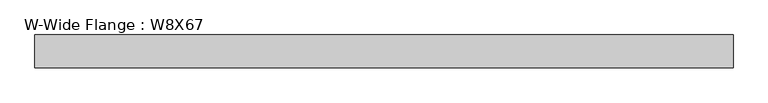
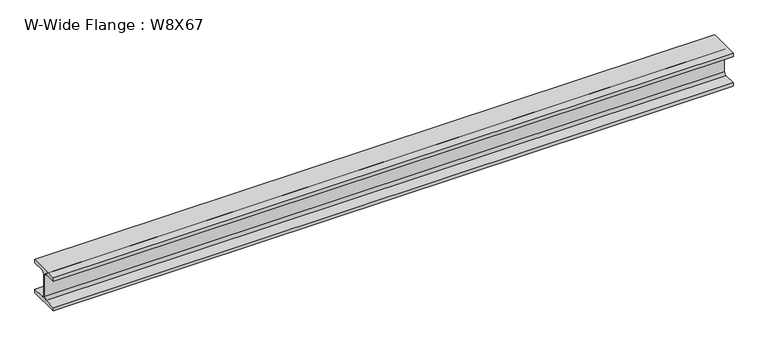
"""IFC4 building model written with IfcOpenShell, lengths in millimetres: beam geometry, W-Wide Flange : W8X67."""

import ifcopenshell
import ifcopenshell.guid

model = None  # the IFC model being written
_history = None  # IfcOwnerHistory: only IFC2X3 demands one
_inside = {}  # id of a spatial element -> (the spatial element, [elements in it])
_under = {}  # id of a project, library or spatial element -> (it, [spatial elements below it])
_declared = {}  # id of a project -> (the project, [libraries it declares])
_typed = {}  # id of a type object -> (the type object, [elements of that type])
_made_of = {}  # id of a material, layer set ... -> (it, [elements and type objects made of it])


def new_model(schema):
    """Start an empty IFC model of exactly this schema.

    Asked for "IFC4X3", IfcOpenShell would pick the latest addendum, in which some entities
    have other attributes; the version numbers below select the first issue.
    IFC2X3 requires an IfcOwnerHistory on every rooted entity: one is made here for all.
    """
    global model, _history
    if schema == "IFC4X3":
        model = ifcopenshell.file(schema_version=(4, 3, 0, 0))
    else:
        model = ifcopenshell.file(schema=schema)
    _inside.clear()
    _under.clear()
    _declared.clear()
    _typed.clear()
    _made_of.clear()
    _history = None
    if model.schema == "IFC2X3":
        org = make("IfcOrganization", Name="unknown")
        user = make(
            "IfcPersonAndOrganization",
            ThePerson=make("IfcPerson", FamilyName="unknown"),
            TheOrganization=org,
        )
        app = make(
            "IfcApplication",
            ApplicationDeveloper=org,
            Version="unknown",
            ApplicationFullName="unknown",
            ApplicationIdentifier="unknown",
        )
        _history = make(
            "IfcOwnerHistory",
            OwningUser=user,
            OwningApplication=app,
            ChangeAction="ADDED",
            CreationDate=0,
        )
    return model


def make(cls, **values):
    """One entity of the class cls with the attributes given. An attribute that is None is left unset."""
    return model.create_entity(
        cls, **{name: value for name, value in values.items() if value is not None}
    )


def rooted(cls, **values):
    """An entity with a GlobalId (a new one), such as an element, a storey or a relation."""
    return make(cls, GlobalId=ifcopenshell.guid.new(), OwnerHistory=_history, **values)


def si_unit(unit_type, name, prefix=None):
    """IfcSIUnit, for example si_unit("LENGTHUNIT", "METRE", prefix="MILLI")."""
    return make("IfcSIUnit", UnitType=unit_type, Prefix=prefix, Name=name)


def assignment(units):
    """IfcUnitAssignment: the units of a project."""
    return None if units is None else make("IfcUnitAssignment", Units=units)


def point(xyz):
    """IfcCartesianPoint."""
    return None if xyz is None else make("IfcCartesianPoint", Coordinates=xyz)


def direction(xyz):
    """IfcDirection."""
    return None if xyz is None else make("IfcDirection", DirectionRatios=xyz)


def frame(location, z_axis=None, x_axis=None):
    """IfcAxis2Placement3D, a coordinate frame: its origin and axes. An axis left out is left unset."""
    return make(
        "IfcAxis2Placement3D",
        Location=point(location),
        Axis=direction(z_axis),
        RefDirection=direction(x_axis),
    )


def frame_2d(location, x_axis=None):
    """IfcAxis2Placement2D, a coordinate frame in the plane: its origin and x axis."""
    return make(
        "IfcAxis2Placement2D", Location=point(location), RefDirection=direction(x_axis)
    )


def origin():
    """The frame at (0, 0, 0) with its axes left unset."""
    return frame((0.0, 0.0, 0.0))


def place(relative_to, where):
    """IfcLocalPlacement: puts the frame where relative to a parent placement (None: the world)."""
    return make(
        "IfcLocalPlacement", PlacementRelTo=relative_to, RelativePlacement=where
    )


def context(
    kind, dimensions, precision=None, world=None, true_north=None, identifier=None
):
    """IfcGeometricRepresentationContext, for example the 3D "Model" context."""
    return make(
        "IfcGeometricRepresentationContext",
        ContextIdentifier=identifier,
        ContextType=kind,
        CoordinateSpaceDimension=dimensions,
        Precision=precision,
        WorldCoordinateSystem=world,
        TrueNorth=true_north,
    )


def project(units=None, contexts=None):
    """IfcProject with its units and contexts."""
    return rooted(
        "IfcProject",
        Name="project",
        RepresentationContexts=contexts,
        UnitsInContext=assignment(units),
    )


def spatial(cls, under=None, at=None, **own):
    """A site, building, storey or space (cls), placed at a placement, below another one or the project."""
    s = rooted(cls, ObjectPlacement=at, **own)
    if under is not None:
        _under.setdefault(under.id(), (under, []))[1].append(s)
    return s


def polyline(points):
    """IfcPolyline through the points."""
    return make("IfcPolyline", Points=[point(p) for p in points])


def circle_curve(where, radius):
    """IfcCircle in the frame where."""
    return make("IfcCircle", Position=where, Radius=radius)


def trimmed(basis, trim1, trim2, sense, master):
    """IfcTrimmedCurve: the piece of a basis curve between two trims."""
    return make(
        "IfcTrimmedCurve",
        BasisCurve=basis,
        Trim1=trim1,
        Trim2=trim2,
        SenseAgreement=sense,
        MasterRepresentation=master,
    )


def segment(curve, same_sense, transition):
    """IfcCompositeCurveSegment."""
    return make(
        "IfcCompositeCurveSegment",
        Transition=transition,
        SameSense=same_sense,
        ParentCurve=curve,
    )


def composite_curve(segments, self_intersect=None):
    """IfcCompositeCurve: segments joined end to end."""
    return make("IfcCompositeCurve", Segments=segments, SelfIntersect=self_intersect)


def outline(outer, holes=None, kind="AREA"):
    """IfcArbitraryClosedProfileDef: a profile drawn as a closed curve; with holes, ...WithVoids."""
    if holes is None:
        return make("IfcArbitraryClosedProfileDef", ProfileType=kind, OuterCurve=outer)
    return make(
        "IfcArbitraryProfileDefWithVoids",
        ProfileType=kind,
        OuterCurve=outer,
        InnerCurves=holes,
    )


def extrude(swept, where, along, depth):
    """IfcExtrudedAreaSolid: the profile swept, set in the frame where, extruded along a direction by depth."""
    return make(
        "IfcExtrudedAreaSolid",
        SweptArea=swept,
        Position=where,
        ExtrudedDirection=direction(along),
        Depth=depth,
    )


def shape(context_of_items, identifier, shape_type, items):
    """IfcShapeRepresentation: the items that make up one representation, for example the "Body"."""
    return make(
        "IfcShapeRepresentation",
        ContextOfItems=context_of_items,
        RepresentationIdentifier=identifier,
        RepresentationType=shape_type,
        Items=items,
    )


def source(mapping_origin, context_of_items, identifier, shape_type, items):
    """IfcRepresentationMap: a shape defined once, which mapped items show again and again."""
    return make(
        "IfcRepresentationMap",
        MappingOrigin=mapping_origin,
        MappedRepresentation=shape(context_of_items, identifier, shape_type, items),
    )


def transform(
    local_origin,
    x_axis=None,
    y_axis=None,
    z_axis=None,
    scale=None,
    scale2=None,
    scale3=None,
    uniform=True,
):
    """IfcCartesianTransformationOperator3D, or its non-uniform kind. x_axis, y_axis, z_axis: its Axis1, 2, 3."""
    if uniform:
        return make(
            "IfcCartesianTransformationOperator3D",
            Axis1=direction(x_axis),
            Axis2=direction(y_axis),
            LocalOrigin=point(local_origin),
            Scale=scale,
            Axis3=direction(z_axis),
        )
    return make(
        "IfcCartesianTransformationOperator3DnonUniform",
        Axis1=direction(x_axis),
        Axis2=direction(y_axis),
        LocalOrigin=point(local_origin),
        Scale=scale,
        Axis3=direction(z_axis),
        Scale2=scale2,
        Scale3=scale3,
    )


def mapped(mapping_source, mapping_target):
    """IfcMappedItem: shows the shape of a source again, moved by a transform."""
    return make(
        "IfcMappedItem", MappingSource=mapping_source, MappingTarget=mapping_target
    )


def made_of(thing, what):
    """Note that an element or type object is made of a material, layer set ...; save() writes the relation."""
    if what is not None:
        _made_of.setdefault(what.id(), (what, []))[1].append(thing)
    return thing


def element(
    cls,
    number,
    at=None,
    inside=None,
    cuts=None,
    type_object=None,
    material=None,
    context=None,
    identifier="Body",
    shape_type=None,
    held_by="IfcProductDefinitionShape",
    body=None,
    shapes=None,
    **own,
):
    """One element of the class cls, such as IfcWall. Its Tag is "e" and its number.

    at: its placement. inside: the storey or other place that contains it. cuts: it is an
    opening in that element (IfcRelVoidsElement). A single representation is given by context,
    identifier, shape_type and body (its items); several are given by shapes. held_by: the class
    of the entity that holds the representations. save() writes the other relations.
    """
    e = rooted(cls, Tag="e%d" % number, ObjectPlacement=at, **own)
    if body is not None:
        shapes = [shape(context, identifier, shape_type, body)]
    if shapes is not None:
        e.Representation = make(held_by, Representations=shapes)
    if inside is not None:
        _inside.setdefault(inside.id(), (inside, []))[1].append(e)
    if cuts is not None:
        rooted(
            "IfcRelVoidsElement", RelatingBuildingElement=cuts, RelatedOpeningElement=e
        )
    if type_object is not None:
        _typed.setdefault(type_object.id(), (type_object, []))[1].append(e)
    return made_of(e, material)


def aggregate(whole, parts):
    """IfcRelAggregates: a whole, such as a stair, and the parts it consists of."""
    return rooted("IfcRelAggregates", RelatingObject=whole, RelatedObjects=parts)


def save(model, path):
    """Write the relations noted so far, then the file.

    IfcRelAggregates (storeys below a building ...), IfcRelContainedInSpatialStructure (elements
    in a storey), IfcRelDefinesByType, IfcRelAssociatesMaterial and IfcRelDeclares: one each for
    every whole, place, type object, material and project.
    """
    for whole, parts in _under.values():
        aggregate(whole, parts)
    for where, things in _inside.values():
        rooted(
            "IfcRelContainedInSpatialStructure",
            RelatedElements=things,
            RelatingStructure=where,
        )
    for kind, things in _typed.values():
        rooted("IfcRelDefinesByType", RelatedObjects=things, RelatingType=kind)
    for what, things in _made_of.values():
        rooted("IfcRelAssociatesMaterial", RelatedObjects=things, RelatingMaterial=what)
    for by, libraries in _declared.values():
        rooted("IfcRelDeclares", RelatingContext=by, RelatedDefinitions=libraries)
    model.write(path)


def w_wide_flange_w8x67_7d7912c2(model_context):
    return source(origin(), model_context, "Body", "SweptSolid", [
        extrude(outline(composite_curve([segment(polyline([(105.156, -90.551), (105.156, -114.3), (-105.156, -114.3), (-105.156, -90.551), (-24.765, -90.551)]), True, "CONTINUOUS"), segment(trimmed(circle_curve(frame_2d((-24.765, -73.025)), 17.526), [point((-24.765, -90.551))], [point((-7.239, -73.025))], True, "CARTESIAN"), True, "CONTINUOUS"), segment(polyline([(-7.239, -73.025), (-7.239, 73.025)]), True, "CONTINUOUS"), segment(trimmed(circle_curve(frame_2d((-24.765, 73.025)), 17.526), [point((-7.239, 73.025))], [point((-24.765, 90.551))], True, "CARTESIAN"), True, "CONTINUOUS"), segment(polyline([(-24.765, 90.551), (-105.156, 90.551), (-105.156, 114.3), (105.156, 114.3), (105.156, 90.551), (24.765, 90.551)]), True, "CONTINUOUS"), segment(trimmed(circle_curve(frame_2d((24.765, 73.025)), 17.526), [point((24.765, 90.551))], [point((7.239, 73.025))], True, "CARTESIAN"), True, "CONTINUOUS"), segment(polyline([(7.239, 73.025), (7.239, -73.025)]), True, "CONTINUOUS"), segment(trimmed(circle_curve(frame_2d((24.765, -73.025)), 17.526), [point((7.239, -73.025))], [point((24.765, -90.551))], True, "CARTESIAN"), True, "CONTINUOUS"), segment(polyline([(24.765, -90.551), (105.156, -90.551)]), True, "CONTINUOUS")], self_intersect=False)), frame((-2228.85, 0.0, 0.0), z_axis=(1.0, 0.0, 0.0), x_axis=(0.0, 1.0, 0.0)), (0.0, 0.0, 1.0), 4444.9999994),
    ])


if __name__ == "__main__":
    model = new_model("IFC4")
    model_context = context("Model", 3, world=origin())
    ifc_project = project(units=[si_unit("LENGTHUNIT", "METRE", prefix="MILLI")], contexts=[model_context])
    site = spatial("IfcSite", under=ifc_project)
    building = spatial("IfcBuilding", under=site)
    placement = place(None, origin())
    w_wide_flange_w8x67_shape = w_wide_flange_w8x67_7d7912c2(model_context)
    element("IfcBeam", 1, ObjectType="W-Wide Flange : W8X67", at=placement, inside=building, context=model_context, shape_type="MappedRepresentation", body=[
        mapped(w_wide_flange_w8x67_shape, transform((0.0, 0.0, 0.0), x_axis=(1.0, 0.0, 0.0), y_axis=(0.0, 1.0, 0.0), z_axis=(0.0, 0.0, 1.0))),
    ])
    save(model, "model.ifc")

# Revit data of these elements
# Type "W-Wide Flange : W8X67"
#   Assembly Code = "B10"
#   W = 67
#   Length [instance default] = 5' - 0"
#   bf = 0' - 8.28"
#   d = 0' - 9"
#   k = 0' - 1 5/8"
#   k2 = 0' - 0.69"
#   tf = 0' - 0.935"
#   tw = 0' - 0.57"
#   A = 0.136806 SF
#   Structural Material [instance default] = _STRUCTURAL STEEL (SEE STRUCT. DWGS)
# Element 1 (IfcBeam, "W-Wide Flange : W8X67")
#   Materials on its faces: "_STRUCTURAL STEEL (SEE STRUCT. DWGS)"
# Materials
#   "_STRUCTURAL STEEL (SEE STRUCT. DWGS)": class "Metal", colour RGB 199 199 199, transparency 0, Description = "Structural steel 50ksi", Cost = 0
